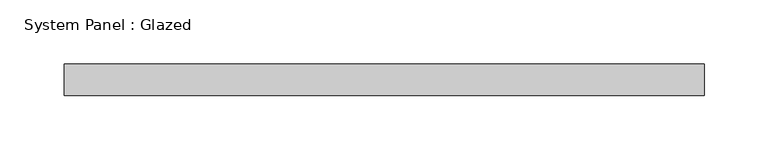
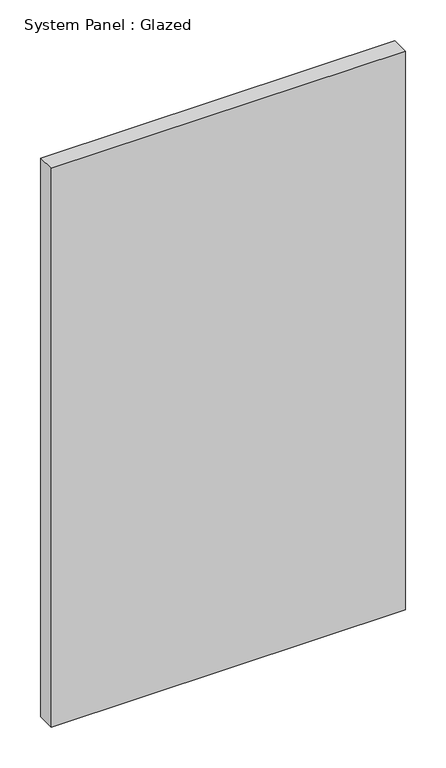
"""IFC4 building model written with IfcOpenShell, lengths in millimetres: plate geometry, System Panel : Glazed."""

from ifc_helpers import new_model, si_unit, origin, origin_with_axes, place, context, project, spatial, polyline, outline, extrude, source, transform, mapped, element, save


def system_panel_glazed_66530992(model_context):
    return source(origin(), model_context, "Body", "SweptSolid", [
        extrude(outline(polyline([(250.0, 24.5), (-250.0, 24.5), (-250.0, 49.5), (250.0, 49.5), (250.0, 24.5)])), origin_with_axes(), (0.0, 0.0, 1.0), 833.3333333),
    ])


if __name__ == "__main__":
    model = new_model("IFC4")
    model_context = context("Model", 3, world=origin())
    ifc_project = project(units=[si_unit("LENGTHUNIT", "METRE", prefix="MILLI")], contexts=[model_context])
    site = spatial("IfcSite", under=ifc_project)
    building = spatial("IfcBuilding", under=site)
    placement = place(None, origin())
    system_panel_glazed_shape = system_panel_glazed_66530992(model_context)
    element("IfcPlate", 1, ObjectType="System Panel : Glazed", at=placement, inside=building, context=model_context, shape_type="MappedRepresentation", body=[
        mapped(system_panel_glazed_shape, transform((0.0, 0.0, 0.0), x_axis=(1.0, 0.0, 0.0), y_axis=(0.0, 1.0, 0.0), z_axis=(0.0, 0.0, 1.0))),
    ])
    save(model, "model.ifc")

# Revit data of these elements
# Element 1 (IfcPlate, "System Panel : Glazed")
#   Materials on its faces: "Glass"
# Materials
#   "Glass": class "Glass", colour RGB 218 227 224, transparency 0.85, Description = "Soda Lime Glass", Cost = 0
